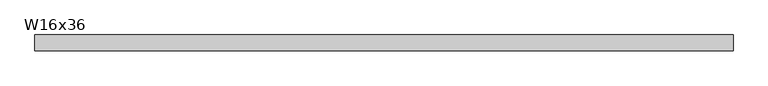
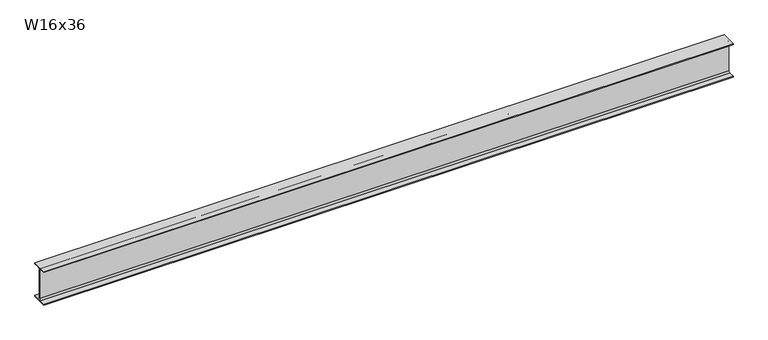
"""IFC4 building model written with IfcOpenShell, lengths in millimetres: beam geometry, RME W-Wide Flange : W16x36."""

from ifc_helpers import new_model, si_unit, point, frame, frame_2d, origin, place, context, project, spatial, polyline, circle_curve, trimmed, segment, composite_curve, outline, extrude, source, transform, mapped, element, save


def w16x36_6e94cf69(model_context):
    return source(origin(), model_context, "Body", "SweptSolid", [
        extrude(outline(composite_curve([segment(polyline([(88.773, -191.008), (88.773, -201.93), (-88.773, -201.93), (-88.773, -191.008), (-21.3995, -191.008)]), True, "CONTINUOUS"), segment(trimmed(circle_curve(frame_2d((-21.3995, -173.355)), 17.653), [point((-21.3995, -191.008))], [point((-3.7465, -173.355))], True, "CARTESIAN"), True, "CONTINUOUS"), segment(polyline([(-3.7465, -173.355), (-3.7465, 173.355)]), True, "CONTINUOUS"), segment(trimmed(circle_curve(frame_2d((-21.3995, 173.355)), 17.653), [point((-3.7465, 173.355))], [point((-21.3995, 191.008))], True, "CARTESIAN"), True, "CONTINUOUS"), segment(polyline([(-21.3995, 191.008), (-88.773, 191.008), (-88.773, 201.93), (88.773, 201.93), (88.773, 191.008), (21.3995, 191.008)]), True, "CONTINUOUS"), segment(trimmed(circle_curve(frame_2d((21.3995, 173.355)), 17.653), [point((21.3995, 191.008))], [point((3.7465, 173.355))], True, "CARTESIAN"), True, "CONTINUOUS"), segment(polyline([(3.7465, 173.355), (3.7465, -173.355)]), True, "CONTINUOUS"), segment(trimmed(circle_curve(frame_2d((21.3995, -173.355)), 17.653), [point((3.7465, -173.355))], [point((21.3995, -191.008))], True, "CARTESIAN"), True, "CONTINUOUS"), segment(polyline([(21.3995, -191.008), (88.773, -191.008)]), True, "CONTINUOUS")], self_intersect=False)), frame((-3962.4, 0.0, 0.0), z_axis=(1.0, 0.0, 0.0), x_axis=(0.0, 1.0, 0.0)), (0.0, 0.0, 1.0), 7864.7688575),
    ])


if __name__ == "__main__":
    model = new_model("IFC4")
    model_context = context("Model", 3, world=origin())
    ifc_project = project(units=[si_unit("LENGTHUNIT", "METRE", prefix="MILLI")], contexts=[model_context])
    site = spatial("IfcSite", under=ifc_project)
    building = spatial("IfcBuilding", under=site)
    placement = place(None, origin())
    w16x36_shape = w16x36_6e94cf69(model_context)
    element("IfcBeam", 1, ObjectType="RME W-Wide Flange : W16x36", at=placement, inside=building, context=model_context, shape_type="MappedRepresentation", body=[
        mapped(w16x36_shape, transform((0.0, 0.0, 0.0), x_axis=(1.0, 0.0, 0.0), y_axis=(0.0, 1.0, 0.0), z_axis=(0.0, 0.0, 1.0))),
    ])
    save(model, "model.ifc")

# Revit data of these elements
# Type "RME W-Wide Flange : W16x36"
#   WELD P [instance default] = ""
#   WELD LE [instance default] = ""
#   WELD D [instance default] = ""
#   TOP SECTION SIZE [instance default] = ""
#   TOP SECTION LENGTH [instance default] = ""
#   REMARKS [instance default] = ""
#   REINF TYPE [instance default] = ""
#   Nominal Size = "W24"
#   End Bearing Capacity [instance default] = ""
#   BOT SECTION SIZE [instance default] = ""
#   BOT SECTION LENGTH [instance default] = ""
#   Assembly Code = "B10"
#   W = 36
#   Start Extension Calculation [instance default] = 10' - 0"
#   Start Extension [instance default] = -0' - 0 1/2"
#   End Extension Calculation [instance default] = 10' - 0"
#   End Extension [instance default] = -0' - 0 1/2"
#   Length [instance default] = 5' - 0"
#   bf = 0' - 6.99"
#   d = 1' - 3.9"
#   k = 0' - 1 1/8"
#   k2 = 0' - 0.695"
#   tf = 0' - 0.43"
#   tw = 0' - 0.295"
#   A = 0.0736111 SF
#   Structural Material [instance default] = Metal - Steel - ASTM A992
# Element 1 (IfcBeam, "RME W-Wide Flange : W16x36")
#   End Extension Calculation = 9' - 9.63657"
#   End Extension = -0' - 2.86343"
#   Length = 26' - 0"
#   Materials on its faces: "Metal - Steel - ASTM A992"
# Materials
#   "Metal - Steel - ASTM A992": class "Metal", colour RGB 255 128 0, transparency 0
